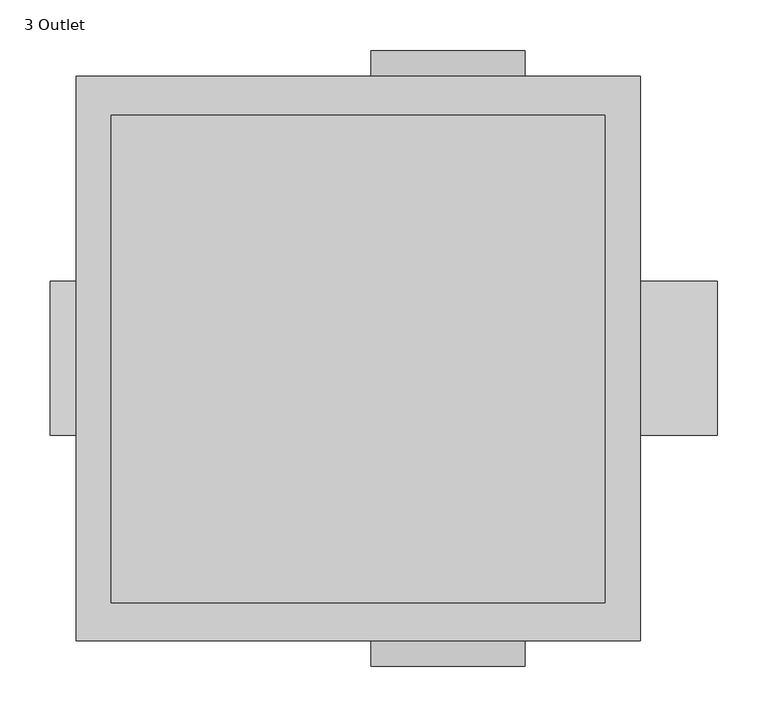
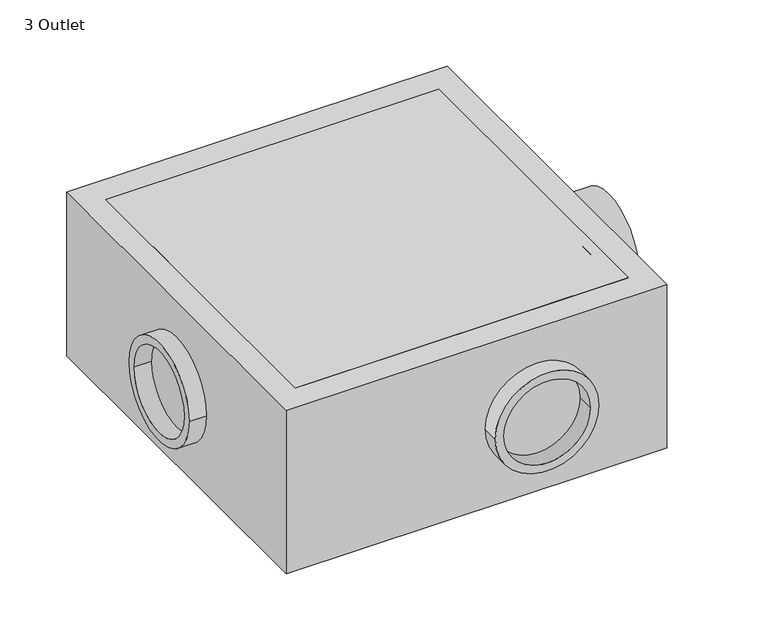
"""IFC4 building model written with IfcOpenShell, lengths in millimetres: geographic element geometry, Septic_Dist-Box : 3 Outlet."""

from ifc_helpers import new_model, si_unit, point, frame, frame_2d, origin, origin_with_axes, place, context, project, spatial, polyline, circle_curve, trimmed, segment, composite_curve, outline, extrude, source, transform, mapped, element, save


def geographic_element_3_outlet_11af9c1a(model_context):
    return source(origin(), model_context, "Body", "SweptSolid", [
        extrude(outline(polyline([(244.4514858, 228.6), (244.4514858, -228.6), (-244.4985142, -228.6), (-244.4985142, 228.6), (244.4514858, 228.6)])), origin_with_axes(), (0.0, 0.0, 1.0), 25.4),
        extrude(outline(composite_curve([segment(trimmed(circle_curve(frame_2d((0.0, 122.3585937)), 76.2), [point((76.2, 122.3585937))], [point((-76.2, 122.3585937))], False, "CARTESIAN"), True, "CONTINUOUS"), segment(trimmed(circle_curve(frame_2d((0.0, 122.3585937)), 76.2), [point((-76.2, 122.3585937))], [point((76.2, 122.3585937))], False, "CARTESIAN"), True, "CONTINUOUS")], self_intersect=False), holes=[composite_curve([segment(trimmed(circle_curve(frame_2d((0.0, 122.3585937)), 63.5), [point((63.5, 122.3585937))], [point((-63.5, 122.3585937))], True, "CARTESIAN"), True, "CONTINUOUS"), segment(trimmed(circle_curve(frame_2d((0.0, 122.3585937)), 63.5), [point((-63.5, 122.3585937))], [point((63.5, 122.3585937))], True, "CARTESIAN"), True, "CONTINUOUS")], self_intersect=False)]), frame((279.4, 0.0, 0.0), z_axis=(1.0, 0.0, 0.0), x_axis=(0.0, 1.0, 0.0)), (0.0, 0.0, 1.0), 76.2),
        extrude(outline(composite_curve([segment(trimmed(circle_curve(frame_2d((0.0, 122.3585937)), 76.2), [point((76.2, 122.3585937))], [point((-76.2, 122.3585937))], False, "CARTESIAN"), True, "CONTINUOUS"), segment(trimmed(circle_curve(frame_2d((0.0, 122.3585937)), 76.2), [point((-76.2, 122.3585937))], [point((76.2, 122.3585937))], False, "CARTESIAN"), True, "CONTINUOUS")], self_intersect=False), holes=[composite_curve([segment(trimmed(circle_curve(frame_2d((0.0, 122.3585937)), 63.5), [point((63.5, 122.3585937))], [point((-63.5, 122.3585937))], True, "CARTESIAN"), True, "CONTINUOUS"), segment(trimmed(circle_curve(frame_2d((0.0, 122.3585937)), 63.5), [point((-63.5, 122.3585937))], [point((63.5, 122.3585937))], True, "CARTESIAN"), True, "CONTINUOUS")], self_intersect=False)]), frame((-304.8, 0.0, 0.0), z_axis=(1.0, 0.0, 0.0), x_axis=(0.0, 1.0, 0.0)), (0.0, 0.0, 1.0), 25.4),
        extrude(outline(composite_curve([segment(trimmed(circle_curve(frame_2d((122.3585937, 88.9)), 76.2), [point((122.3585937, 165.1))], [point((122.3585937, 12.7))], False, "CARTESIAN"), True, "CONTINUOUS"), segment(trimmed(circle_curve(frame_2d((122.3585937, 88.9)), 76.2), [point((122.3585937, 12.7))], [point((122.3585937, 165.1))], False, "CARTESIAN"), True, "CONTINUOUS")], self_intersect=False), holes=[composite_curve([segment(trimmed(circle_curve(frame_2d((122.3585937, 88.9)), 63.5), [point((122.3585937, 152.4))], [point((122.3585937, 25.4))], True, "CARTESIAN"), True, "CONTINUOUS"), segment(trimmed(circle_curve(frame_2d((122.3585937, 88.9)), 63.5), [point((122.3585937, 25.4))], [point((122.3585937, 152.4))], True, "CARTESIAN"), True, "CONTINUOUS")], self_intersect=False)]), frame((0.0, 279.4, 0.0), z_axis=(0.0, 1.0, 0.0), x_axis=(0.0, 0.0, 1.0)), (0.0, 0.0, 1.0), 25.4),
        extrude(outline(composite_curve([segment(trimmed(circle_curve(frame_2d((122.3585937, 88.9)), 76.2), [point((122.3585937, 165.1))], [point((122.3585937, 12.7))], False, "CARTESIAN"), True, "CONTINUOUS"), segment(trimmed(circle_curve(frame_2d((122.3585937, 88.9)), 76.2), [point((122.3585937, 12.7))], [point((122.3585937, 165.1))], False, "CARTESIAN"), True, "CONTINUOUS")], self_intersect=False), holes=[composite_curve([segment(trimmed(circle_curve(frame_2d((122.3585937, 88.9)), 63.5), [point((122.3585937, 152.4))], [point((122.3585937, 25.4))], True, "CARTESIAN"), True, "CONTINUOUS"), segment(trimmed(circle_curve(frame_2d((122.3585937, 88.9)), 63.5), [point((122.3585937, 25.4))], [point((122.3585937, 152.4))], True, "CARTESIAN"), True, "CONTINUOUS")], self_intersect=False)]), frame((0.0, -304.8, 0.0), z_axis=(0.0, 1.0, 0.0), x_axis=(0.0, 0.0, 1.0)), (0.0, 0.0, 1.0), 25.4),
        extrude(outline(polyline([(244.4514858, 240.6542817), (244.4514858, -241.9457183), (-244.4985142, -241.9457183), (-244.4985142, 240.6542817), (244.4514858, 240.6542817)])), frame((0.0, 0.0, 228.6), z_axis=(0.0, 0.0, 1.0), x_axis=(1.0, 0.0, 0.0)), (0.0, 0.0, 1.0), 25.4),
        extrude(outline(polyline([(279.4, 279.4), (279.4, -279.4), (-279.4, -279.4), (-279.4, 279.4), (279.4, 279.4)]), holes=[polyline([(-228.6, -228.6), (228.6, -228.6), (228.6, 228.6), (-228.6, 228.6), (-228.6, -228.6)])]), origin_with_axes(), (0.0, 0.0, 1.0), 254.0),
    ])


if __name__ == "__main__":
    model = new_model("IFC4")
    model_context = context("Model", 3, world=origin())
    ifc_project = project(units=[si_unit("LENGTHUNIT", "METRE", prefix="MILLI")], contexts=[model_context])
    site = spatial("IfcSite", under=ifc_project)
    building = spatial("IfcBuilding", under=site)
    placement = place(None, origin())
    geographic_element_3_outlet_shape = geographic_element_3_outlet_11af9c1a(model_context)
    element("IfcGeographicElement", 1, ObjectType="Septic_Dist-Box : 3 Outlet", at=placement, inside=building, context=model_context, shape_type="MappedRepresentation", body=[
        mapped(geographic_element_3_outlet_shape, transform((0.0, 0.0, 0.0), x_axis=(1.0, 0.0, 0.0), y_axis=(0.0, 1.0, 0.0), z_axis=(0.0, 0.0, 1.0))),
    ])
    save(model, "model.ifc")

# Revit data of these elements
# Type "Septic_Dist-Box : 3 Outlet"
#   COBie.Type.CreatedBy = "design@eagle.com"
#   COBie.Type.CreatedOn = "2016-10-27T05:31:12"
#   COBie.Type.Name = "Septic_Dist-Box_3 Outlet"
#   COBie.Type.Category = "23-70 50 14 21 : Septic Tank Systems"
#   COBie.Type.Description = "Septic_Dist-Box_3 Outlet"
#   COBie.Type.Manufacturer = "Generic"
#   COBie.Type.ModelNumber = "Generic"
#   Test Data = ""
#   Specification = "http://www.arcat.com/divs/sec/sec02540.shtml"
#   Sales Information = ""
#   Product Properties = "http://www.arcat.com/bim/bim_info.pl?fn=Septic_Dist-Box"
#   Product Data = "http://www.arcat.com/divs/sec/sec02540.shtml"
#   Model = "Generic"
#   Manufacturer Website = "http://www.arcat.com/"
#   Manufacturer Phone - Toll Free = ""
#   Manufacturer Phone = "(203) 929-9444"
#   Manufacturer Fax = "(203) 939-2444"
#   Manufacturer Email = "bim@arcat.com"
#   Manufacturer Address = "1077 Bridgeport Ave, Shelton, CT  06484"
#   Manufacturer = "Generic"
#   Keynote = "02540"
#   Installation_Fabricaton = ""
#   Installation Phase = ""
#   Green Building-LEED = "http://www.arcat.com/green/green_building.shtml"
#   Drawn By = "Robert S. Weygant. CSI, CDT, SCIP"
#   Description = "Septic Distribution Box - 3 Outlet"
#   Copyright = "2008, ARCAT, Inc."
#   Construction Details = "http://www.arcat.com/divs/sec/sec02540.shtml"
#   Building Codes = ""
#   Assembly Code = "G3020300"
#   COBie.Type.ReplacementCost = 0
#   od = 0' - 3"
#   id = 0' - 2 1/2"
#   Width = 1' - 10"
#   Outlet Diameter = 0' - 5"
#   Length = 1' - 10"
#   Depth Below Grade = 0' - 11"
#   Depth = 0' - 10"
#   COBie.Type = yes
#   Warranty Duration (Years) = 0
#   Max Outlets = 3
#   Outlets = 3
#   Maintenance Schedule (Months) = 0
#   Expected Lifespan (Years) = 0
#   3 = yes
#   2 = no
#   1 = yes
#   Site Metalwork Trim = ARCAT - Metal - Steel, Painted - Green
#   Site Metalwork Material = ARCAT - Metal - Steel, Painted - Black
#   Site Metalwork Accent = ARCAT - Metal - Steel, Painted - Brown
#   Body Material = ARCAT - Concrete - Precast_6000psi
# Element 1 (IfcGeographicElement, "Septic_Dist-Box : 3 Outlet")
#   Materials on its faces: "ARCAT - Concrete - Precast_6000psi"
# Materials
#   "ARCAT - Metal - Steel, Painted - Green": class "Unassigned", colour RGB 27 114 27, transparency 0, Model = "Generic", Manufacturer = "Generic", Description = "Steel, Painted"
#   "ARCAT - Metal - Steel, Painted - Black": class "Unassigned", colour RGB 0 0 0, transparency 0, Model = "Generic", Manufacturer = "Generic", Description = "Steel, Painted"
#   "ARCAT - Metal - Steel, Painted - Brown": class "Unassigned", colour RGB 104 81 55, transparency 0, Model = "Generic", Manufacturer = "Generic", Description = "Steel, Painted"
#   "ARCAT - Concrete - Precast_6000psi": class "Unassigned", colour RGB 198 187 187, transparency 0, Keynote = "03410", Model = "Generic", Manufacturer = "Generic", Description = "6000psi Precast Concrete"
